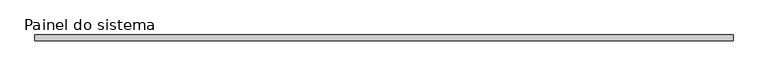
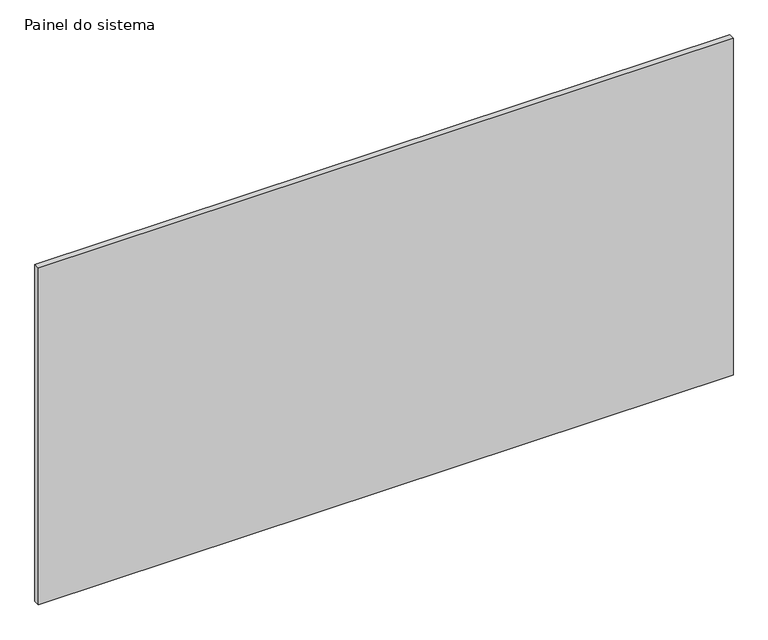
"""IFC4 building model written with IfcOpenShell, lengths in millimetres: plate geometry, Painel do sistema : Envidraçado."""

from ifc_helpers import new_model, si_unit, origin, origin_with_axes, place, context, project, spatial, polyline, outline, extrude, source, transform, mapped, element, save


def painel_do_sistema_af596b93(model_context):
    return source(origin(), model_context, "Body", "SweptSolid", [
        extrude(outline(polyline([(1462.4999925, 24.5), (-1462.4999925, 24.5), (-1462.4999925, 49.5), (1462.4999925, 49.5), (1462.4999925, 24.5)])), origin_with_axes(), (0.0, 0.0, 1.0), 1500.0),
    ])


if __name__ == "__main__":
    model = new_model("IFC4")
    model_context = context("Model", 3, world=origin())
    ifc_project = project(units=[si_unit("LENGTHUNIT", "METRE", prefix="MILLI")], contexts=[model_context])
    site = spatial("IfcSite", under=ifc_project)
    building = spatial("IfcBuilding", under=site)
    placement = place(None, origin())
    painel_do_sistema_shape = painel_do_sistema_af596b93(model_context)
    element("IfcPlate", 1, ObjectType="Painel do sistema : Envidraçado", at=placement, inside=building, context=model_context, shape_type="MappedRepresentation", body=[
        mapped(painel_do_sistema_shape, transform((0.0, 0.0, 0.0), x_axis=(1.0, 0.0, 0.0), y_axis=(0.0, 1.0, 0.0), z_axis=(0.0, 0.0, 1.0))),
    ])
    save(model, "model.ifc")

# Revit data of these elements
# Type "Painel do sistema : Envidraçado"
#   Construction Type Id = "GSP4R"
#   Analytic Construction = "Vidraça única Pilkington 1/8 pol"
#   Visual Light Transmittance = 0.9
#   Solar Heat Gain Coefficient = 0.86
#   Heat Transfer Coefficient (U) = 6.7069 W/(m²·K)
# Element 1 (IfcPlate, "Painel do sistema : Envidraçado")
#   Materials on its faces: "Vidro"
# Materials
#   "Vidro": class "Vidro", colour RGB 0 128 192, transparency 0.9, Description = "Vidro de sílica", Cost = 0
